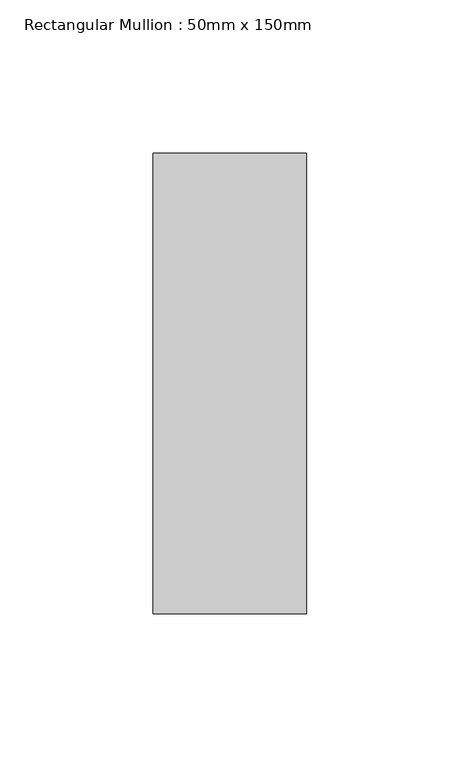
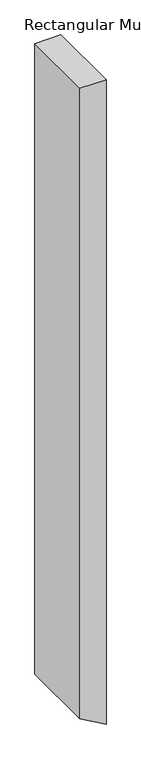
"""IFC4 building model written with IfcOpenShell, lengths in millimetres: member geometry, Rectangular Mullion : 50mm x 150mm."""

from ifc_helpers import new_model, si_unit, frame, origin, place, context, project, spatial, polyline, outline, extrude, source, transform, mapped, element, save


def rectangular_mullion_50mm_x_150mm_ea3fe943(model_context):
    return source(origin(), model_context, "Body", "SweptSolid", [
        extrude(outline(polyline([(0.0, 25.0), (0.0, -25.0), (-1280.5229345, -25.0), (-1309.3904479, 25.0), (0.0, 25.0)])), frame((0.0, -75.0, 0.0), z_axis=(0.0, 1.0, 0.0), x_axis=(0.0, 0.0, 1.0)), (0.0, 0.0, 1.0), 150.0),
    ])


if __name__ == "__main__":
    model = new_model("IFC4")
    model_context = context("Model", 3, world=origin())
    ifc_project = project(units=[si_unit("LENGTHUNIT", "METRE", prefix="MILLI")], contexts=[model_context])
    site = spatial("IfcSite", under=ifc_project)
    building = spatial("IfcBuilding", under=site)
    placement = place(None, origin())
    rectangular_mullion_50mm_x_150mm_shape = rectangular_mullion_50mm_x_150mm_ea3fe943(model_context)
    element("IfcMember", 1, ObjectType="Rectangular Mullion : 50mm x 150mm", at=placement, inside=building, context=model_context, shape_type="MappedRepresentation", body=[
        mapped(rectangular_mullion_50mm_x_150mm_shape, transform((0.0, 0.0, 0.0), x_axis=(1.0, 0.0, 0.0), y_axis=(0.0, 1.0, 0.0), z_axis=(0.0, 0.0, 1.0))),
    ])
    save(model, "model.ifc")

# Revit data of these elements
# Type "Rectangular Mullion : 50mm x 150mm"
#   built-in parameter 1007304 = 0.492126 (stored number, unit not read)
#   built-in parameter 1007301 = 0.082021 (stored number, unit not read)
#   built-in parameter 1007300 = 0.082021 (stored number, unit not read)
# Element 1 (IfcMember, "Rectangular Mullion : 50mm x 150mm")
#   Materials on its faces: "Aluminum"
# Materials
#   "Aluminum": class "Metal", colour RGB 247 247 247, transparency 0, Description = "Aluminum 6061", Cost = 0
